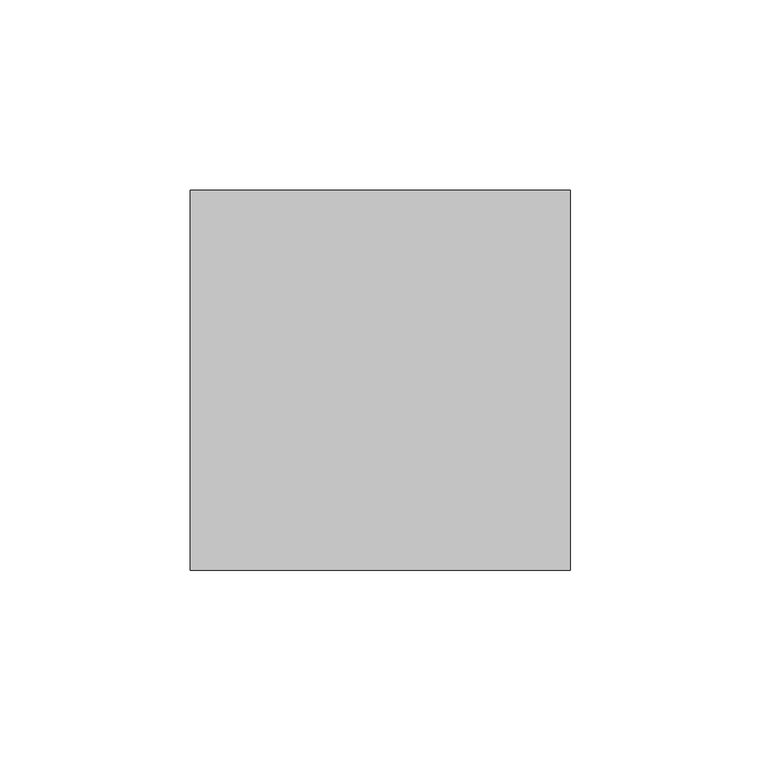
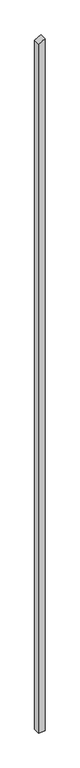
"""IFC4 building model written with IfcOpenShell, lengths in millimetres: column geometry, Holzstütze 158756 : Holzstütze 158756."""

from ifc_helpers import new_model, si_unit, frame, origin, place, context, project, spatial, polyline, outline, extrude, source, transform, mapped, element, save


def column_c7102fa8(model_context):
    return source(origin(), model_context, "Body", "SweptSolid", [
        extrude(outline(polyline([(-500.0, 165627.7593015), (-500.0, 165727.7593015), (10641.011365, 165727.7593015), (10590.0588201, 165627.7593015), (-500.0, 165627.7593015)])), frame((0.0, 47884.7962965, 0.0), z_axis=(0.0, 1.0, 0.0), x_axis=(0.0, 0.0, 1.0)), (0.0, 0.0, 1.0), 100.0),
    ])


if __name__ == "__main__":
    model = new_model("IFC4")
    model_context = context("Model", 3, world=origin())
    ifc_project = project(units=[si_unit("LENGTHUNIT", "METRE", prefix="MILLI")], contexts=[model_context])
    site = spatial("IfcSite", under=ifc_project)
    building = spatial("IfcBuilding", under=site)
    placement = place(None, origin())
    column_shape = column_c7102fa8(model_context)
    element("IfcColumn", 1, ObjectType="Holzstütze 158756 : Holzstütze 158756", at=placement, inside=building, context=model_context, shape_type="MappedRepresentation", body=[
        mapped(column_shape, transform((0.0, 0.0, 0.0), x_axis=(1.0, 0.0, 0.0), y_axis=(0.0, 1.0, 0.0), z_axis=(0.0, 0.0, 1.0))),
    ])
    save(model, "model.ifc")

# Revit data of these elements
# Type "Holzstütze 158756 : Holzstütze 158756"
#   Abrechnungsart = "m"
#   Allright_Bauteil_ID = "0152St 0000143526"
#   Bezeichnung = "Holzstütze"
#   Codetext = "ST-HOLZ\\"
#   Gewerk = "Zimmer- und Holzbauarbeiten"
#   Material = "Holz"
#   Objektname = "Stütze"
#   NameOverride = "Holzstütze"
#   Reference = "Holzstütze"
#   Status = "NEW"
#   ThermalTransmittance = 0.0000 BTU/(h·ft²·°F)
#   Roll = 0.00°
#   Slope = 0.00°
#   2D Interaktion = yes
#   IsExternal = yes
#   LoadBearing = yes
# Element 1 (IfcColumn, "Holzstütze 158756 : Holzstütze 158756")
#   Materials on its faces: "holzschalung"
# Materials
#   "holzschalung": class "Unassigned", colour RGB 128 128 128, transparency 0
